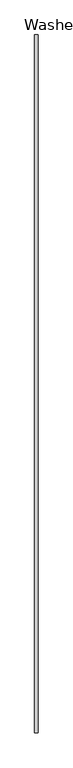
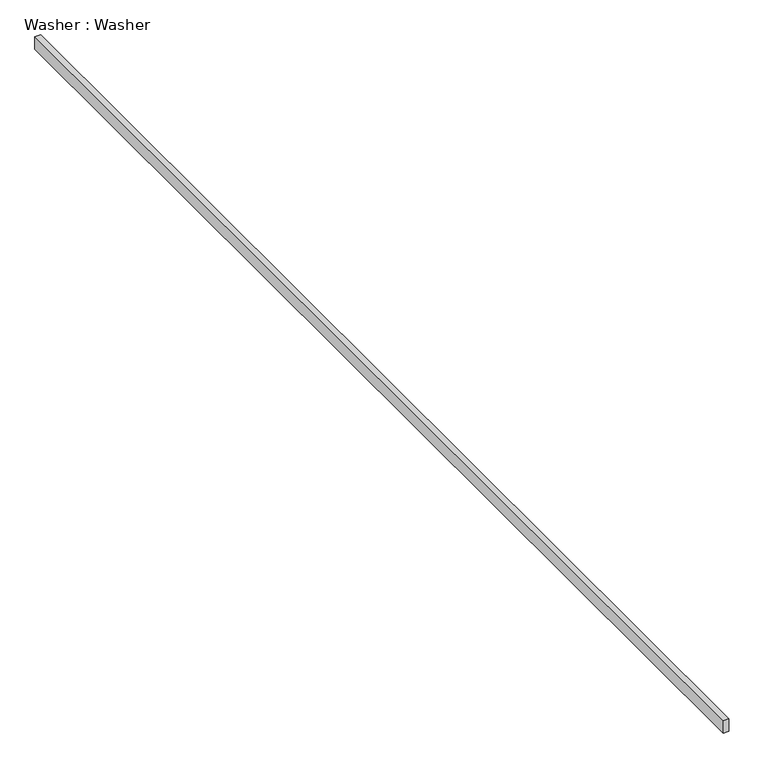
"""IFC4 building model written with IfcOpenShell, lengths in millimetres: proxy geometry, Washer : Washer."""

from ifc_helpers import new_model, si_unit, frame, origin, place, context, project, spatial, polyline, outline, extrude, source, transform, mapped, element, save


def washer_washer_985b0542(model_context):
    return source(origin(), model_context, "Body", "SweptSolid", [
        extrude(outline(polyline([(-7093.2617633, 7982.1531721), (-7102.7867633, 7982.1531721), (-7102.7867633, 9982.1531721), (-7093.2617633, 9982.1531721), (-7093.2617633, 7982.1531721)])), frame((0.0, 0.0, 40153.9643859), z_axis=(0.0, 0.0, 1.0), x_axis=(1.0, 0.0, 0.0)), (0.0, 0.0, 1.0), 22.1367188),
    ])


if __name__ == "__main__":
    model = new_model("IFC4")
    model_context = context("Model", 3, world=origin())
    ifc_project = project(units=[si_unit("LENGTHUNIT", "METRE", prefix="MILLI")], contexts=[model_context])
    site = spatial("IfcSite", under=ifc_project)
    building = spatial("IfcBuilding", under=site)
    placement = place(None, origin())
    washer_washer_shape = washer_washer_985b0542(model_context)
    element("IfcBuildingElementProxy", 1, Name="Washer : Washer", ObjectType="Washer : Washer", at=placement, inside=building, context=model_context, shape_type="MappedRepresentation", body=[
        mapped(washer_washer_shape, transform((0.0, 0.0, 0.0), x_axis=(1.0, 0.0, 0.0), y_axis=(0.0, 1.0, 0.0), z_axis=(0.0, 0.0, 1.0))),
    ])
    save(model, "model.ifc")

# Revit data of these elements
# Type "Washer : Washer"
#   NameOverride = "Washer"
# Element 1 (IfcBuildingElementProxy, "Washer : Washer")
#   Materials on its faces: "GASKETED WASHER FOR DRAINAGE"
# Materials
#   "GASKETED WASHER FOR DRAINAGE": class "Unassigned", colour RGB 128 128 128, transparency 0
